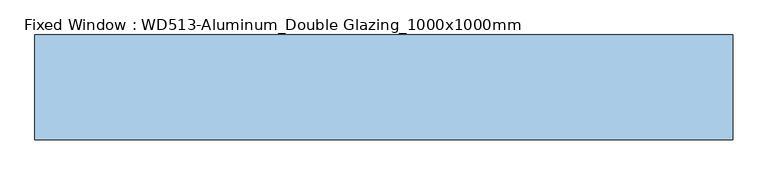
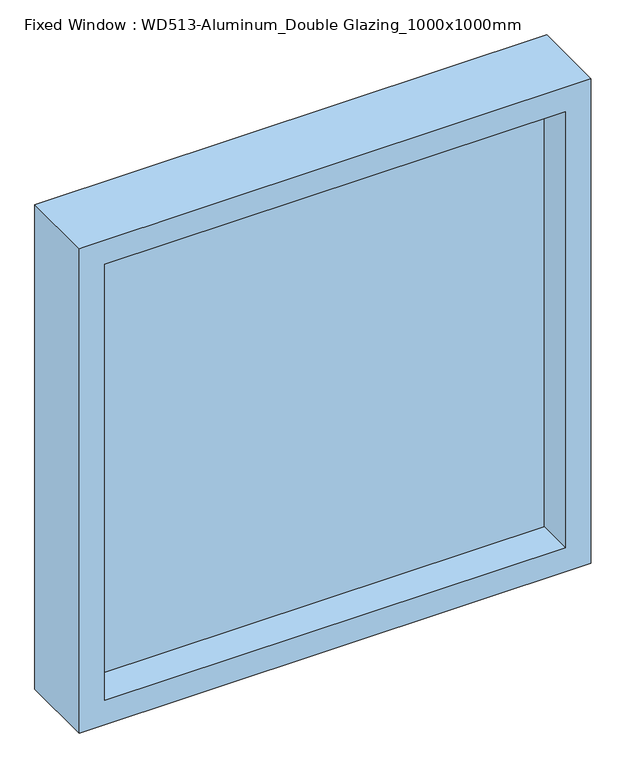
"""IFC4 building model written with IfcOpenShell, lengths in millimetres: window geometry, Fixed Window : WD513-Aluminum_Double Glazing_1000x1000mm."""

from ifc_helpers import new_model, si_unit, frame, origin, place, context, project, spatial, polyline, outline, extrude, source, transform, mapped, element, save


def fixed_window_wd513_aluminum_double_glazing_1000x1000mm_e073f05b(model_context):
    return source(origin(), model_context, "Body", "SweptSolid", [
        extrude(outline(polyline([(-450.0, 3.0), (450.0, 3.0), (450.0, -3.0), (-450.0, -3.0), (-450.0, 3.0)])), frame((0.0, 0.0, 850.0), z_axis=(0.0, 0.0, 1.0), x_axis=(1.0, 0.0, 0.0)), (0.0, 0.0, 1.0), 900.0),
        extrude(outline(polyline([(1800.0, -500.0), (800.0, -500.0), (800.0, 500.0), (1800.0, 500.0), (1800.0, -500.0)]), holes=[polyline([(1750.0, -450.0), (1750.0, 450.0), (850.0, 450.0), (850.0, -450.0), (1750.0, -450.0)])]), frame((0.0, -75.0, 0.0), z_axis=(0.0, 1.0, 0.0), x_axis=(0.0, 0.0, 1.0)), (0.0, 0.0, 1.0), 150.0),
    ])


if __name__ == "__main__":
    model = new_model("IFC4")
    model_context = context("Model", 3, world=origin())
    ifc_project = project(units=[si_unit("LENGTHUNIT", "METRE", prefix="MILLI")], contexts=[model_context])
    site = spatial("IfcSite", under=ifc_project)
    building = spatial("IfcBuilding", under=site)
    placement = place(None, origin())
    fixed_window_wd513_aluminum_double_glazing_1000x1000mm_shape = fixed_window_wd513_aluminum_double_glazing_1000x1000mm_e073f05b(model_context)
    element("IfcWindow", 1, ObjectType="Fixed Window : WD513-Aluminum_Double Glazing_1000x1000mm", at=placement, inside=building, context=model_context, shape_type="MappedRepresentation", body=[
        mapped(fixed_window_wd513_aluminum_double_glazing_1000x1000mm_shape, transform((0.0, 0.0, 0.0), x_axis=(1.0, 0.0, 0.0), y_axis=(0.0, 1.0, 0.0), z_axis=(0.0, 0.0, 1.0))),
    ])
    save(model, "model.ifc")

# Revit data of these elements
# Type "Fixed Window : WD513-Aluminum_Double Glazing_1000x1000mm"
#   Type Mark = "193"
#   Analytic Construction = "<None>"
#   창 두께 = 150 mm
#   Height = 1000 mm
#   절반 창 두께 = 75 mm
#   기본 씰 높이 = 800 mm
#   Width = 1000 mm
#   Define Thermal Properties by = 1
#   창 패널 = AW2 창 패널
#   창 프레임 = A04AQ127-00002_Aluminum Window_None FP
#   Wall Closure = (empty or 0)
# Element 1 (IfcWindow, "Fixed Window : WD513-Aluminum_Double Glazing_1000x1000mm")
#   Materials on its faces: "A04AQ127-00002_Aluminum Window_None FP", "AW2 창 패널"
# Materials
#   "AW2 창 패널": class "유리", colour RGB 0 0 255, transparency 0.75
#   "A04AQ127-00002_Aluminum Window_None FP": class "금속", colour RGB 247 247 247, transparency 0, W00) Work Master Code = "A04AQ127-00002", W01) Work Master_Lv1 = "Finishing Work", W02) Work Master_Lv2 = "Door & Window Work", W03) Work Master_Spec.1 = "Aluminum Window", W04) Work Master_Spec.2 = "Fire Protective Rating: N/A", W05) Work Master_Spec.3 = "w/ Hardware & Accessories", Cost = 0
